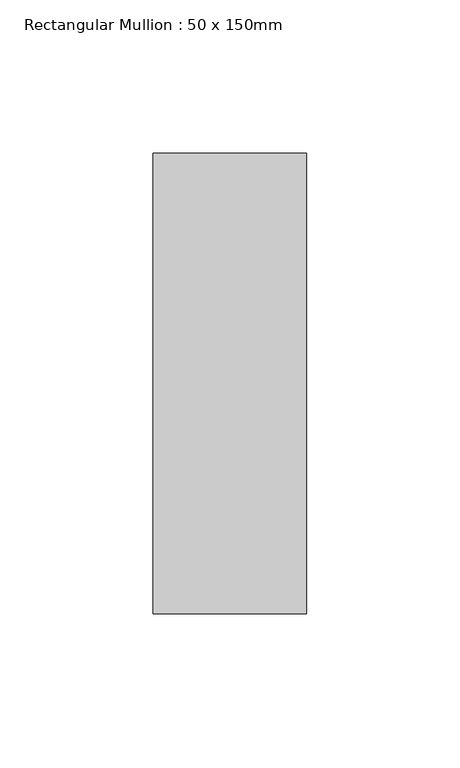
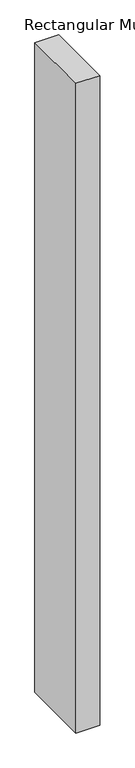
"""IFC4 building model written with IfcOpenShell, lengths in millimetres: member geometry, Rectangular Mullion : 50 x 150mm."""

import ifcopenshell
import ifcopenshell.guid

model = None  # the IFC model being written
_history = None  # IfcOwnerHistory: only IFC2X3 demands one
_inside = {}  # id of a spatial element -> (the spatial element, [elements in it])
_under = {}  # id of a project, library or spatial element -> (it, [spatial elements below it])
_declared = {}  # id of a project -> (the project, [libraries it declares])
_typed = {}  # id of a type object -> (the type object, [elements of that type])
_made_of = {}  # id of a material, layer set ... -> (it, [elements and type objects made of it])


def new_model(schema):
    """Start an empty IFC model of exactly this schema.

    Asked for "IFC4X3", IfcOpenShell would pick the latest addendum, in which some entities
    have other attributes; the version numbers below select the first issue.
    IFC2X3 requires an IfcOwnerHistory on every rooted entity: one is made here for all.
    """
    global model, _history
    if schema == "IFC4X3":
        model = ifcopenshell.file(schema_version=(4, 3, 0, 0))
    else:
        model = ifcopenshell.file(schema=schema)
    _inside.clear()
    _under.clear()
    _declared.clear()
    _typed.clear()
    _made_of.clear()
    _history = None
    if model.schema == "IFC2X3":
        org = make("IfcOrganization", Name="unknown")
        user = make(
            "IfcPersonAndOrganization",
            ThePerson=make("IfcPerson", FamilyName="unknown"),
            TheOrganization=org,
        )
        app = make(
            "IfcApplication",
            ApplicationDeveloper=org,
            Version="unknown",
            ApplicationFullName="unknown",
            ApplicationIdentifier="unknown",
        )
        _history = make(
            "IfcOwnerHistory",
            OwningUser=user,
            OwningApplication=app,
            ChangeAction="ADDED",
            CreationDate=0,
        )
    return model


def make(cls, **values):
    """One entity of the class cls with the attributes given. An attribute that is None is left unset."""
    return model.create_entity(
        cls, **{name: value for name, value in values.items() if value is not None}
    )


def rooted(cls, **values):
    """An entity with a GlobalId (a new one), such as an element, a storey or a relation."""
    return make(cls, GlobalId=ifcopenshell.guid.new(), OwnerHistory=_history, **values)


def si_unit(unit_type, name, prefix=None):
    """IfcSIUnit, for example si_unit("LENGTHUNIT", "METRE", prefix="MILLI")."""
    return make("IfcSIUnit", UnitType=unit_type, Prefix=prefix, Name=name)


def assignment(units):
    """IfcUnitAssignment: the units of a project."""
    return None if units is None else make("IfcUnitAssignment", Units=units)


def point(xyz):
    """IfcCartesianPoint."""
    return None if xyz is None else make("IfcCartesianPoint", Coordinates=xyz)


def direction(xyz):
    """IfcDirection."""
    return None if xyz is None else make("IfcDirection", DirectionRatios=xyz)


def frame(location, z_axis=None, x_axis=None):
    """IfcAxis2Placement3D, a coordinate frame: its origin and axes. An axis left out is left unset."""
    return make(
        "IfcAxis2Placement3D",
        Location=point(location),
        Axis=direction(z_axis),
        RefDirection=direction(x_axis),
    )


def origin():
    """The frame at (0, 0, 0) with its axes left unset."""
    return frame((0.0, 0.0, 0.0))


def place(relative_to, where):
    """IfcLocalPlacement: puts the frame where relative to a parent placement (None: the world)."""
    return make(
        "IfcLocalPlacement", PlacementRelTo=relative_to, RelativePlacement=where
    )


def context(
    kind, dimensions, precision=None, world=None, true_north=None, identifier=None
):
    """IfcGeometricRepresentationContext, for example the 3D "Model" context."""
    return make(
        "IfcGeometricRepresentationContext",
        ContextIdentifier=identifier,
        ContextType=kind,
        CoordinateSpaceDimension=dimensions,
        Precision=precision,
        WorldCoordinateSystem=world,
        TrueNorth=true_north,
    )


def project(units=None, contexts=None):
    """IfcProject with its units and contexts."""
    return rooted(
        "IfcProject",
        Name="project",
        RepresentationContexts=contexts,
        UnitsInContext=assignment(units),
    )


def spatial(cls, under=None, at=None, **own):
    """A site, building, storey or space (cls), placed at a placement, below another one or the project."""
    s = rooted(cls, ObjectPlacement=at, **own)
    if under is not None:
        _under.setdefault(under.id(), (under, []))[1].append(s)
    return s


def polyline(points):
    """IfcPolyline through the points."""
    return make("IfcPolyline", Points=[point(p) for p in points])


def outline(outer, holes=None, kind="AREA"):
    """IfcArbitraryClosedProfileDef: a profile drawn as a closed curve; with holes, ...WithVoids."""
    if holes is None:
        return make("IfcArbitraryClosedProfileDef", ProfileType=kind, OuterCurve=outer)
    return make(
        "IfcArbitraryProfileDefWithVoids",
        ProfileType=kind,
        OuterCurve=outer,
        InnerCurves=holes,
    )


def extrude(swept, where, along, depth):
    """IfcExtrudedAreaSolid: the profile swept, set in the frame where, extruded along a direction by depth."""
    return make(
        "IfcExtrudedAreaSolid",
        SweptArea=swept,
        Position=where,
        ExtrudedDirection=direction(along),
        Depth=depth,
    )


def shape(context_of_items, identifier, shape_type, items):
    """IfcShapeRepresentation: the items that make up one representation, for example the "Body"."""
    return make(
        "IfcShapeRepresentation",
        ContextOfItems=context_of_items,
        RepresentationIdentifier=identifier,
        RepresentationType=shape_type,
        Items=items,
    )


def source(mapping_origin, context_of_items, identifier, shape_type, items):
    """IfcRepresentationMap: a shape defined once, which mapped items show again and again."""
    return make(
        "IfcRepresentationMap",
        MappingOrigin=mapping_origin,
        MappedRepresentation=shape(context_of_items, identifier, shape_type, items),
    )


def transform(
    local_origin,
    x_axis=None,
    y_axis=None,
    z_axis=None,
    scale=None,
    scale2=None,
    scale3=None,
    uniform=True,
):
    """IfcCartesianTransformationOperator3D, or its non-uniform kind. x_axis, y_axis, z_axis: its Axis1, 2, 3."""
    if uniform:
        return make(
            "IfcCartesianTransformationOperator3D",
            Axis1=direction(x_axis),
            Axis2=direction(y_axis),
            LocalOrigin=point(local_origin),
            Scale=scale,
            Axis3=direction(z_axis),
        )
    return make(
        "IfcCartesianTransformationOperator3DnonUniform",
        Axis1=direction(x_axis),
        Axis2=direction(y_axis),
        LocalOrigin=point(local_origin),
        Scale=scale,
        Axis3=direction(z_axis),
        Scale2=scale2,
        Scale3=scale3,
    )


def mapped(mapping_source, mapping_target):
    """IfcMappedItem: shows the shape of a source again, moved by a transform."""
    return make(
        "IfcMappedItem", MappingSource=mapping_source, MappingTarget=mapping_target
    )


def made_of(thing, what):
    """Note that an element or type object is made of a material, layer set ...; save() writes the relation."""
    if what is not None:
        _made_of.setdefault(what.id(), (what, []))[1].append(thing)
    return thing


def element(
    cls,
    number,
    at=None,
    inside=None,
    cuts=None,
    type_object=None,
    material=None,
    context=None,
    identifier="Body",
    shape_type=None,
    held_by="IfcProductDefinitionShape",
    body=None,
    shapes=None,
    **own,
):
    """One element of the class cls, such as IfcWall. Its Tag is "e" and its number.

    at: its placement. inside: the storey or other place that contains it. cuts: it is an
    opening in that element (IfcRelVoidsElement). A single representation is given by context,
    identifier, shape_type and body (its items); several are given by shapes. held_by: the class
    of the entity that holds the representations. save() writes the other relations.
    """
    e = rooted(cls, Tag="e%d" % number, ObjectPlacement=at, **own)
    if body is not None:
        shapes = [shape(context, identifier, shape_type, body)]
    if shapes is not None:
        e.Representation = make(held_by, Representations=shapes)
    if inside is not None:
        _inside.setdefault(inside.id(), (inside, []))[1].append(e)
    if cuts is not None:
        rooted(
            "IfcRelVoidsElement", RelatingBuildingElement=cuts, RelatedOpeningElement=e
        )
    if type_object is not None:
        _typed.setdefault(type_object.id(), (type_object, []))[1].append(e)
    return made_of(e, material)


def aggregate(whole, parts):
    """IfcRelAggregates: a whole, such as a stair, and the parts it consists of."""
    return rooted("IfcRelAggregates", RelatingObject=whole, RelatedObjects=parts)


def save(model, path):
    """Write the relations noted so far, then the file.

    IfcRelAggregates (storeys below a building ...), IfcRelContainedInSpatialStructure (elements
    in a storey), IfcRelDefinesByType, IfcRelAssociatesMaterial and IfcRelDeclares: one each for
    every whole, place, type object, material and project.
    """
    for whole, parts in _under.values():
        aggregate(whole, parts)
    for where, things in _inside.values():
        rooted(
            "IfcRelContainedInSpatialStructure",
            RelatedElements=things,
            RelatingStructure=where,
        )
    for kind, things in _typed.values():
        rooted("IfcRelDefinesByType", RelatedObjects=things, RelatingType=kind)
    for what, things in _made_of.values():
        rooted("IfcRelAssociatesMaterial", RelatedObjects=things, RelatingMaterial=what)
    for by, libraries in _declared.values():
        rooted("IfcRelDeclares", RelatingContext=by, RelatedDefinitions=libraries)
    model.write(path)


def rectangular_mullion_50_x_150mm_1344d69d(model_context):
    return source(origin(), model_context, "Body", "SweptSolid", [
        extrude(outline(polyline([(0.0, 75.0), (0.0, -75.0), (-50.0, -75.0), (-50.0, 75.0), (0.0, 75.0)])), frame((0.0, 0.0, -1450.1029933), z_axis=(0.0, 0.0, 1.0), x_axis=(1.0, 0.0, 0.0)), (0.0, 0.0, 1.0), 1450.1029933),
    ])


if __name__ == "__main__":
    model = new_model("IFC4")
    model_context = context("Model", 3, world=origin())
    ifc_project = project(units=[si_unit("LENGTHUNIT", "METRE", prefix="MILLI")], contexts=[model_context])
    site = spatial("IfcSite", under=ifc_project)
    building = spatial("IfcBuilding", under=site)
    placement = place(None, origin())
    rectangular_mullion_50_x_150mm_shape = rectangular_mullion_50_x_150mm_1344d69d(model_context)
    element("IfcMember", 1, ObjectType="Rectangular Mullion : 50 x 150mm", at=placement, inside=building, context=model_context, shape_type="MappedRepresentation", body=[
        mapped(rectangular_mullion_50_x_150mm_shape, transform((0.0, 0.0, 0.0), x_axis=(1.0, 0.0, 0.0), y_axis=(0.0, 1.0, 0.0), z_axis=(0.0, 0.0, 1.0))),
    ])
    save(model, "model.ifc")

# Revit data of these elements
# Type "Rectangular Mullion : 50 x 150mm"
#   Keynote = "H11"
#   built-in parameter 1007304 = 0.492126 (stored number, unit not read)
#   built-in parameter 1007301 = 0.082021 (stored number, unit not read)
#   built-in parameter 1007300 = 0.082021 (stored number, unit not read)
# Element 1 (IfcMember, "Rectangular Mullion : 50 x 150mm")
#   Materials on its faces: "Aluminium"
# Materials
#   "Aluminium": class "Metal", colour RGB 247 247 247, transparency 0, Description = "Aluminium 6061", Cost = 0
